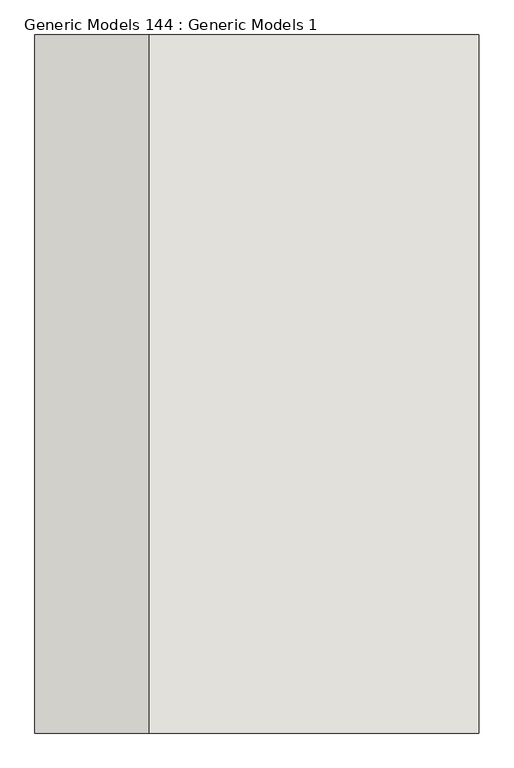
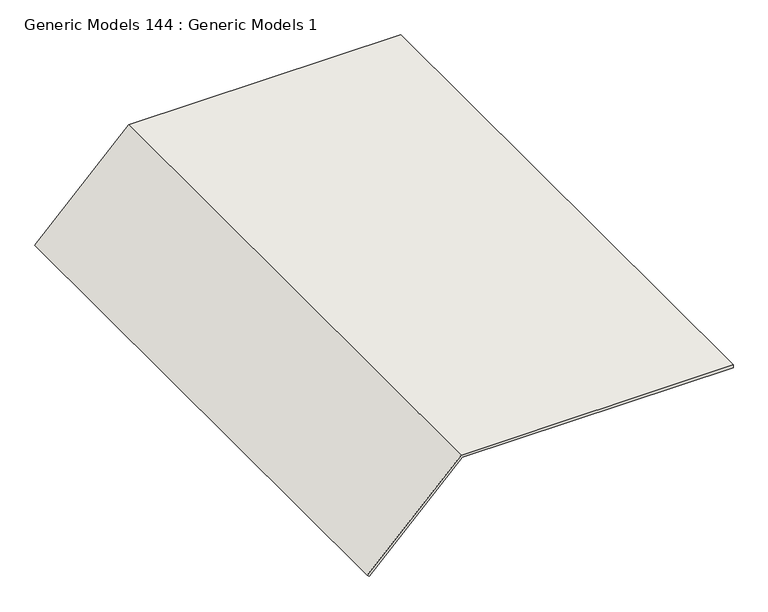
"""IFC4 building model written with IfcOpenShell, lengths in millimetres: wall geometry, Generic Models 144 : Generic Models 1."""

from ifc_helpers import new_model, si_unit, frame, origin, place, context, project, spatial, polyline, outline, extrude, source, transform, mapped, element, save


def generic_models_144_generic_models_1_4ebe4832(model_context):
    return source(origin(), model_context, "Body", "SweptSolid", [
        extrude(outline(polyline([(-79.375, 52785.9625), (-73.025, 52785.9625), (-73.025, 52209.6280698), (-272.1843039, 52010.4687659), (-276.674432, 52014.9588939), (-79.375, 52212.2583259), (-79.375, 52785.9625)])), frame((0.0, 0.0, 0.0), z_axis=(0.0, 1.0, 0.0), x_axis=(0.0, 0.0, 1.0)), (0.0, 0.0, 1.0), 1219.2),
    ])


if __name__ == "__main__":
    model = new_model("IFC4")
    model_context = context("Model", 3, world=origin())
    ifc_project = project(units=[si_unit("LENGTHUNIT", "METRE", prefix="MILLI")], contexts=[model_context])
    site = spatial("IfcSite", under=ifc_project)
    building = spatial("IfcBuilding", under=site)
    placement = place(None, origin())
    generic_models_144_generic_models_1_shape = generic_models_144_generic_models_1_4ebe4832(model_context)
    element("IfcWall", 1, ObjectType="Generic Models 144 : Generic Models 1", at=placement, inside=building, context=model_context, shape_type="MappedRepresentation", body=[
        mapped(generic_models_144_generic_models_1_shape, transform((0.0, 0.0, 0.0), x_axis=(1.0, 0.0, 0.0), y_axis=(0.0, 1.0, 0.0), z_axis=(0.0, 0.0, 1.0))),
    ])
    save(model, "model.ifc")

# Revit data of these elements
# Element 1 (IfcWall, "Generic Models 144 : Generic Models 1")
#   Materials on its faces: "#10 6x6 WIRE MESH"
# Materials
#   "#10 6x6 WIRE MESH": class "Metal", colour RGB 189 187 185, transparency 0, Description = "Structural steel 50ksi", Cost = 0
